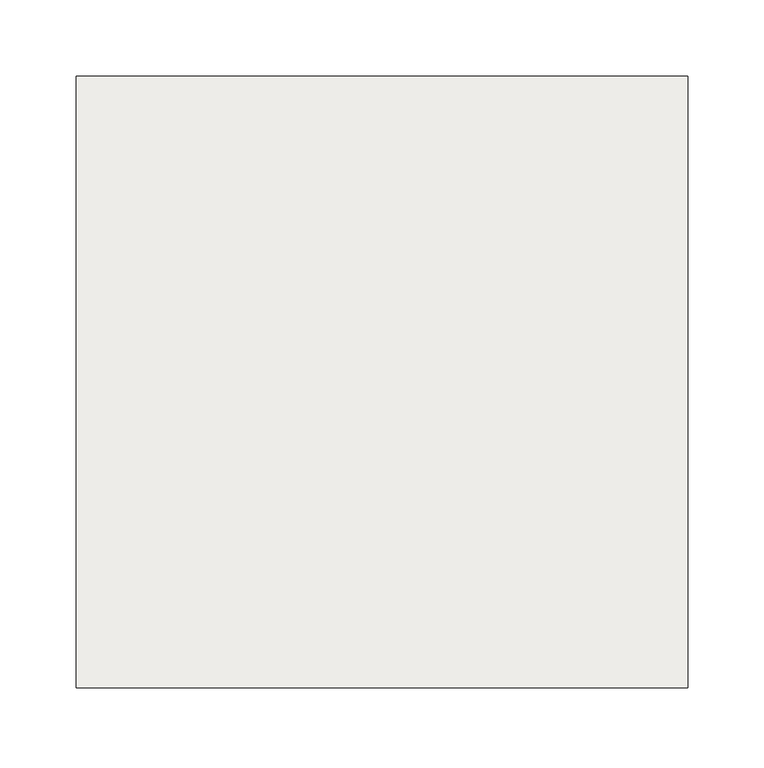
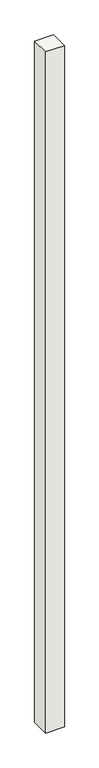
"""IFC4 building model written with IfcOpenShell, lengths in millimetres: footing geometry, NLRS_17_SFO_TLB_funderingspaal geheid beton prefab-AV-MMBPC_gen_rsf : heipaal beton prefab_gen__bxh 400x400."""

from ifc_helpers import new_model, si_unit, frame, origin, place, context, project, spatial, polyline, outline, extrude, source, transform, mapped, element, save


def footing_e3f33549(model_context):
    return source(origin(), model_context, "Body", "SweptSolid", [
        extrude(outline(polyline([(200.0, -200.0), (-200.0, -200.0), (-200.0, 200.0), (200.0, 200.0), (200.0, -200.0)])), frame((0.0, 0.0, -20000.0), z_axis=(0.0, 0.0, 1.0), x_axis=(1.0, 0.0, 0.0)), (0.0, 0.0, 1.0), 15320.0),
    ])


if __name__ == "__main__":
    model = new_model("IFC4")
    model_context = context("Model", 3, world=origin())
    ifc_project = project(units=[si_unit("LENGTHUNIT", "METRE", prefix="MILLI")], contexts=[model_context])
    site = spatial("IfcSite", under=ifc_project)
    building = spatial("IfcBuilding", under=site)
    placement = place(None, origin())
    footing_shape = footing_e3f33549(model_context)
    element("IfcFooting", 1, ObjectType="NLRS_17_SFO_TLB_funderingspaal geheid beton prefab-AV-MMBPC_gen_rsf : heipaal beton prefab_gen__bxh 400x400", at=placement, inside=building, context=model_context, shape_type="MappedRepresentation", body=[
        mapped(footing_shape, transform((0.0, 0.0, 0.0), x_axis=(1.0, 0.0, 0.0), y_axis=(0.0, 1.0, 0.0), z_axis=(0.0, 0.0, 1.0))),
    ])
    save(model, "model.ifc")

# Revit data of these elements
# Type "NLRS_17_SFO_TLB_funderingspaal geheid beton prefab-AV-MMBPC_gen_rsf : heipaal beton prefab_gen__bxh 400x400"
#   IfcExportAs = "IfcPile"
#   Type Comments = "prefab heipaal 400x400"
#   Model = " "
#   Manufacturer = " "
#   Description = "prefab heipaal 400x400"
#   Assembly Code = "17.21"
#   Width = 400 mm
#   Slanted Angle [instance default] = 0.00°
#   NLRS_S_draagvermogen_trek [instance default] = 0.00 kN
#   NLRS_S_draagvermogen_druk [instance default] = 0.00 kN
#   NLRS_C_lengte [instance default] = 1660 mm
#   NLRS_C_hoogte = 400 mm
#   NLRS_C_breedte = 400 mm
#   Height [instance default] = 1660 mm
#   Length [instance default] = 1660 mm
#   Angle [instance default] = 0.00°
#   Slanted [instance default] = 0
#   Structural Material = NLRS_f2_beton prefab_gen_rsf
#   Keynote = ""
# Element 1 (IfcFooting, "NLRS_17_SFO_TLB_funderingspaal geheid beton prefab-AV-MMBPC_gen_rsf : heipaal beton prefab_gen__bxh 400x400")
#   NLRS_C_lengte = 15320 mm
#   Height = 15320 mm
#   Length = 15320 mm
#   Materials on its faces: "NLRS_f2_beton prefab_gen_rsf"
# Materials
#   "NLRS_f2_beton prefab_gen_rsf": class "F - Niet gebakken kunststeen", colour RGB 129 133 118, transparency 0, Keynote = "f2", Manufacturer = "Revit Standards Foundation", URL = "www.revitstandards.org", Description = "beton prefab", Cost = 0
